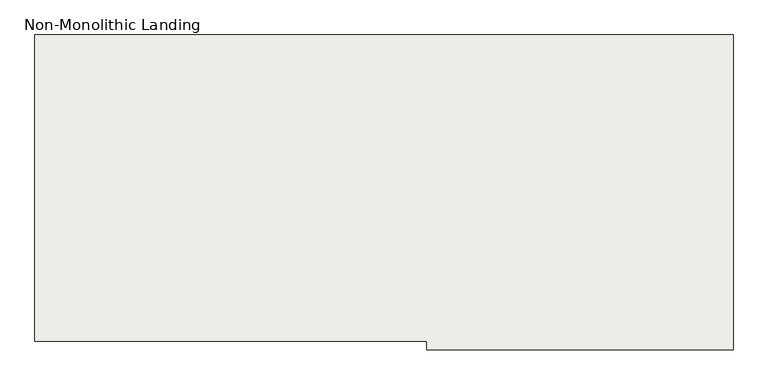
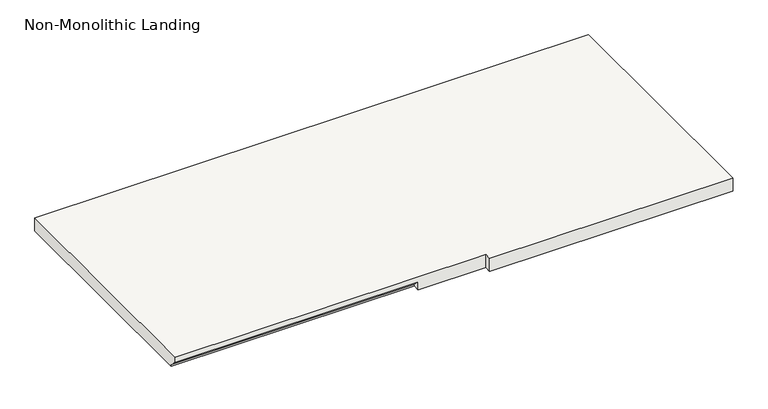
"""IFC4 building model written with IfcOpenShell, lengths in millimetres: slab geometry, Non-Monolithic Landing."""

from ifc_helpers import new_model, si_unit, origin, place, context, project, spatial, faceted_brep, source, transform, mapped, element, save


def non_monolithic_landing_5f150f5a(model_context):
    return source(origin(), model_context, "Body", "Brep", [
        faceted_brep([(16081.5123343, 17121.2483822, 1524.0), (16081.5123343, 17095.8483822, 1524.0), (16995.9123343, 17095.8483822, 1524.0), (16995.9123343, 17121.2483822, 1524.0), (16995.9123343, 18035.6483822, 1524.0), (14913.1123343, 18035.6483822, 1524.0), (14913.1123343, 17121.2483822, 1524.0), (15827.5123343, 17146.6483822, 1473.2), (14913.1123343, 17146.6483822, 1473.2), (14913.1123343, 18035.6483822, 1473.2), (16995.9123343, 18035.6483822, 1473.2), (16995.9123343, 17121.2483822, 1473.2), (16995.9123343, 17095.8483822, 1473.2), (16081.5123343, 17095.8483822, 1473.2), (16081.5123343, 17121.2483822, 1473.2), (15827.5123343, 17121.2483822, 1473.2), (15827.5123343, 17146.6483822, 1479.55), (14913.1123343, 17146.6483822, 1479.55), (15827.5123343, 17121.2483822, 1504.95), (14913.1123343, 17121.2483822, 1504.95)], [[[0, 1, 2, 3, 4, 5, 6]], [[7, 8, 9, 10, 11, 12, 13, 14, 15]], [[8, 7, 16, 17]], [[7, 15, 18, 16]], [[0, 6, 19, 18, 15, 14]], [[1, 0, 14, 13]], [[2, 1, 13, 12]], [[3, 2, 12, 11]], [[4, 3, 11, 10]], [[5, 4, 10, 9]], [[6, 5, 9, 8, 17, 19]], [[19, 17, 16, 18]]]),
    ])


if __name__ == "__main__":
    model = new_model("IFC4")
    model_context = context("Model", 3, world=origin())
    ifc_project = project(units=[si_unit("LENGTHUNIT", "METRE", prefix="MILLI")], contexts=[model_context])
    site = spatial("IfcSite", under=ifc_project)
    building = spatial("IfcBuilding", under=site)
    placement = place(None, origin())
    non_monolithic_landing_shape = non_monolithic_landing_5f150f5a(model_context)
    element("IfcSlab", 1, ObjectType="Non-Monolithic Landing", at=placement, inside=building, context=model_context, shape_type="MappedRepresentation", body=[
        mapped(non_monolithic_landing_shape, transform((0.0, 0.0, 0.0), x_axis=(1.0, 0.0, 0.0), y_axis=(0.0, 1.0, 0.0), z_axis=(0.0, 0.0, 1.0))),
    ])
    save(model, "model.ifc")

# Revit data of these elements
# Element 1 (IfcSlab, "Non-Monolithic Landing")
#   Materials on its faces: "Oak Flooring"
# Materials
#   "Oak Flooring": class "Wood", colour RGB 216 169 114, transparency 0, Description = "Quercus Rubra", Cost = 0
